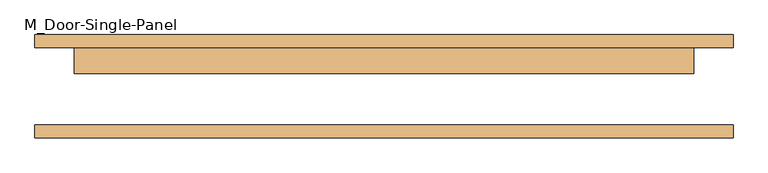
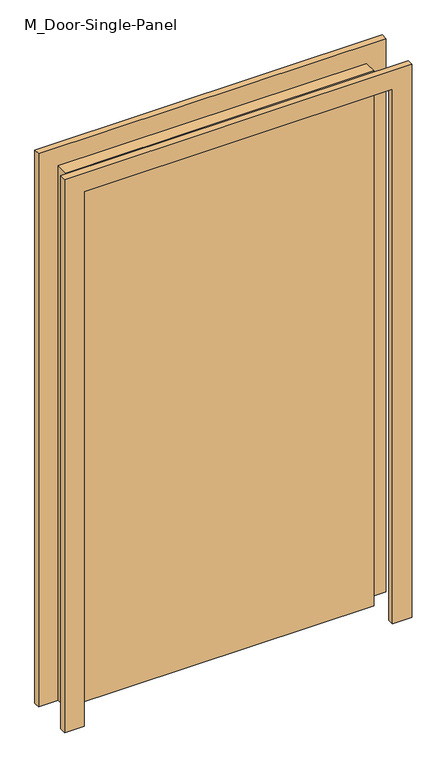
"""IFC4 building model written with IfcOpenShell, lengths in millimetres: door geometry, M_Door-Single-Panel : 1200 x 2200mm DAPC."""

from ifc_helpers import new_model, si_unit, frame, origin, origin_with_axes, place, context, project, spatial, polyline, outline, extrude, source, transform, mapped, element, save


def m_door_single_panel_48f22be7(model_context):
    return source(origin(), model_context, "Body", "SweptSolid", [
        extrude(outline(polyline([(600.0, 25.0), (-600.0, 25.0), (-600.0, 75.0), (600.0, 75.0), (600.0, 25.0)])), origin_with_axes(), (0.0, 0.0, 1.0), 2200.0),
        extrude(outline(polyline([(2276.2, 676.2), (2276.2, -676.2), (0.0, -676.2), (0.0, -600.0), (2200.0, -600.0), (2200.0, 600.0), (0.0, 600.0), (0.0, 676.2), (2276.2, 676.2)])), frame((0.0, -100.0, 0.0), z_axis=(0.0, 1.0, 0.0), x_axis=(0.0, 0.0, 1.0)), (0.0, 0.0, 1.0), 25.0),
        extrude(outline(polyline([(2276.2, -676.2), (0.0, -676.2), (0.0, -600.0), (2200.0, -600.0), (2200.0, 600.0), (0.0, 600.0), (0.0, 676.2), (2276.2, 676.2), (2276.2, -676.2)])), frame((0.0, 75.0, 0.0), z_axis=(0.0, 1.0, 0.0), x_axis=(0.0, 0.0, 1.0)), (0.0, 0.0, 1.0), 25.0),
    ])


if __name__ == "__main__":
    model = new_model("IFC4")
    model_context = context("Model", 3, world=origin())
    ifc_project = project(units=[si_unit("LENGTHUNIT", "METRE", prefix="MILLI")], contexts=[model_context])
    site = spatial("IfcSite", under=ifc_project)
    building = spatial("IfcBuilding", under=site)
    placement = place(None, origin())
    m_door_single_panel_shape = m_door_single_panel_48f22be7(model_context)
    element("IfcDoor", 1, ObjectType="M_Door-Single-Panel : 1200 x 2200mm DAPC", at=placement, inside=building, context=model_context, shape_type="MappedRepresentation", body=[
        mapped(m_door_single_panel_shape, transform((0.0, 0.0, 0.0), x_axis=(1.0, 0.0, 0.0), y_axis=(0.0, 1.0, 0.0), z_axis=(0.0, 0.0, 1.0))),
    ])
    save(model, "model.ifc")

# Revit data of these elements
# Type "M_Door-Single-Panel : 1200 x 2200mm DAPC"
#   Type Mark = "49"
#   Construction Type Id = "DOOR"
#   Analytic Construction = "Wooden"
#   Thickness = 0.05 m
#   Thermal Resistance (R) = 0.455703 (m²·K)/W
#   Swing Angle [instance default] = 90.00°
#   Heat Transfer Coefficient (U) = 2.19465 W/(m²·K)
#   Height = 2.20 m
#   Trim Projection Ext = 0.025 m
#   Trim Projection Int = 0.025 m
#   Trim Width = 0.08 m
#   Width = 1.20 m
#   Define Thermal Properties by = 1
#   Panel Material = Wood - Birch - Solid Stained Light Low Gloss
#   Trim Material = Paint - Sienna
#   Visual Light Transmittance = 0
#   Solar Heat Gain Coefficient = 0
#   Function = (empty or 0)
#   Wall Closure = (empty or 0)
# Element 1 (IfcDoor, "M_Door-Single-Panel : 1200 x 2200mm DAPC")
#   Materials on its faces: "Paint - Sienna", "Wood - Birch - Solid Stained Light Low Gloss"
# Materials
#   "Wood - Birch - Solid Stained Light Low Gloss": class "Wood", colour RGB 210 159 95, transparency 0, Cost = 0
#   "Paint - Sienna": class "Miscellaneous", colour RGB 118 70 51, transparency 0, Cost = 0
